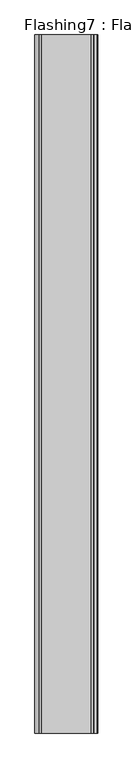
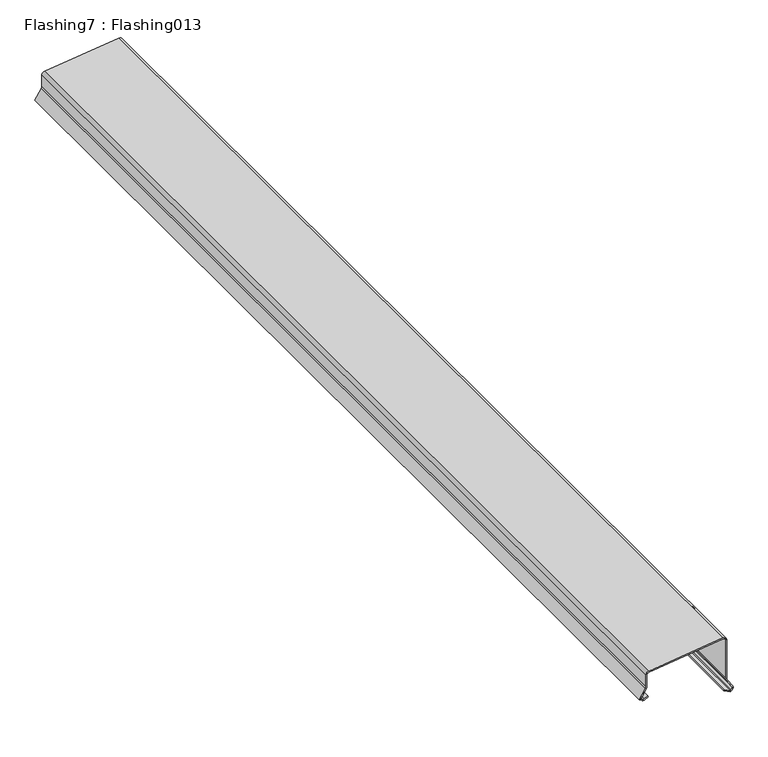
"""IFC4 building model written with IfcOpenShell, lengths in millimetres: proxy geometry, Flashing7 : Flashing013."""

from ifc_helpers import new_model, si_unit, point, frame, frame_2d, origin, place, context, project, spatial, polyline, circle_curve, trimmed, segment, composite_curve, outline, extrude, source, transform, mapped, element, save


def flashing7_flashing013_fca4859d(model_context):
    return source(origin(), model_context, "Body", "SweptSolid", [
        extrude(outline(composite_curve([segment(polyline([(40127.5360053, -9416.8782953), (40130.8867187, -9409.9548736), (40132.6869689, -9410.8261368), (40129.3362554, -9417.7495585)]), True, "CONTINUOUS"), segment(trimmed(circle_curve(frame_2d((40133.2517994, -9419.6445559)), 4.35), [point((40129.3362554, -9417.7495585))], [point((40129.5632143, -9421.9503831))], True, "CARTESIAN"), True, "CONTINUOUS"), segment(polyline([(40129.5632143, -9421.9503831), (40131.5072723, -9425.0602534), (40148.3948046, -9414.1661265)]), True, "CONTINUOUS"), segment(trimmed(circle_curve(frame_2d((40152.9212544, -9421.1828033)), 8.35), [point((40148.3948046, -9414.1661265))], [point((40152.9212544, -9412.8328033))], False, "CARTESIAN"), True, "CONTINUOUS"), segment(polyline([(40152.9212544, -9412.8328033), (40176.1640916, -9412.8328033)]), True, "CONTINUOUS"), segment(trimmed(circle_curve(frame_2d((40176.1640916, -9408.4828033)), 4.35), [point((40176.1640916, -9412.8328033))], [point((40180.4823161, -9409.0076242))], True, "CARTESIAN"), True, "CONTINUOUS"), segment(polyline([(40180.4823161, -9409.0076242), (40197.712243, -9267.2398508)]), True, "CONTINUOUS"), segment(trimmed(circle_curve(frame_2d((40193.3940184, -9266.7150298)), 4.35), [point((40197.712243, -9267.2398508))], [point((40193.3940184, -9262.3650298))], True, "CARTESIAN"), True, "CONTINUOUS"), segment(polyline([(40193.3940184, -9262.3650298), (40116.1659228, -9262.3650299)]), True, "CONTINUOUS"), segment(trimmed(circle_curve(frame_2d((40116.1659228, -9254.0150299)), 8.35), [point((40116.1659228, -9262.3650299))], [point((40111.6503228, -9261.0386939))], False, "CARTESIAN"), True, "CONTINUOUS"), segment(polyline([(40111.6503228, -9261.0386939), (40095.8098632, -9250.8546675)]), True, "CONTINUOUS"), segment(trimmed(circle_curve(frame_2d((40093.4574249, -9254.5137021)), 4.35), [point((40095.8098632, -9250.8546675))], [point((40089.7935443, -9252.1688185))], True, "CARTESIAN"), True, "CONTINUOUS"), segment(polyline([(40089.7935443, -9252.1688185), (40088.63264, -9253.9827315), (40093.9764738, -9264.6739664), (40092.1875, -9265.5681549), (40086.3359375, -9253.8611236), (40088.1090015, -9251.0907111)]), True, "CONTINUOUS"), segment(trimmed(circle_curve(frame_2d((40093.4574249, -9254.5137021)), 6.35), [point((40088.1090015, -9251.0907111))], [point((40096.8914441, -9249.1723528))], False, "CARTESIAN"), True, "CONTINUOUS"), segment(polyline([(40096.8914441, -9249.1723528), (40112.7319037, -9259.3563791)]), True, "CONTINUOUS"), segment(trimmed(circle_curve(frame_2d((40116.1659228, -9254.0150299)), 6.35), [point((40112.7319037, -9259.3563791))], [point((40116.1659228, -9260.3650299))], True, "CARTESIAN"), True, "CONTINUOUS"), segment(polyline([(40116.1659228, -9260.3650299), (40193.3940184, -9260.3650299)]), True, "CONTINUOUS"), segment(trimmed(circle_curve(frame_2d((40193.3940184, -9266.7150299)), 6.35), [point((40193.3940184, -9260.3650299))], [point((40199.6976336, -9267.4811477))], False, "CARTESIAN"), True, "CONTINUOUS"), segment(polyline([(40199.6976336, -9267.4811477), (40182.4677067, -9409.2489212)]), True, "CONTINUOUS"), segment(trimmed(circle_curve(frame_2d((40176.1640916, -9408.4828033)), 6.35), [point((40182.4677067, -9409.2489212))], [point((40176.1640916, -9414.8328033))], False, "CARTESIAN"), True, "CONTINUOUS"), segment(polyline([(40176.1640916, -9414.8328033), (40152.9212544, -9414.8328033)]), True, "CONTINUOUS"), segment(trimmed(circle_curve(frame_2d((40152.9212544, -9421.1828033)), 6.35), [point((40152.9212544, -9414.8328033))], [point((40149.4789842, -9415.8467677))], True, "CARTESIAN"), True, "CONTINUOUS"), segment(polyline([(40149.4789842, -9415.8467677), (40130.8867187, -9427.8406158), (40127.867313, -9423.0105336)]), True, "CONTINUOUS"), segment(trimmed(circle_curve(frame_2d((40133.2517994, -9419.6445559)), 6.35), [point((40127.867313, -9423.0105336))], [point((40127.5360053, -9416.8782953))], False, "CARTESIAN"), True, "CONTINUOUS")], self_intersect=False)), frame((0.0, 7982.1531721, 0.0), z_axis=(0.0, 1.0, 0.0), x_axis=(0.0, 0.0, 1.0)), (0.0, 0.0, 1.0), 2000.0),
    ])


if __name__ == "__main__":
    model = new_model("IFC4")
    model_context = context("Model", 3, world=origin())
    ifc_project = project(units=[si_unit("LENGTHUNIT", "METRE", prefix="MILLI")], contexts=[model_context])
    site = spatial("IfcSite", under=ifc_project)
    building = spatial("IfcBuilding", under=site)
    placement = place(None, origin())
    flashing7_flashing013_shape = flashing7_flashing013_fca4859d(model_context)
    element("IfcBuildingElementProxy", 1, Name="Flashing7 : Flashing013", ObjectType="Flashing7 : Flashing013", at=placement, inside=building, context=model_context, shape_type="MappedRepresentation", body=[
        mapped(flashing7_flashing013_shape, transform((0.0, 0.0, 0.0), x_axis=(1.0, 0.0, 0.0), y_axis=(0.0, 1.0, 0.0), z_axis=(0.0, 0.0, 1.0))),
    ])
    save(model, "model.ifc")

# Revit data of these elements
# Type "Flashing7 : Flashing013"
#   NameOverride = "Flashing013"
# Element 1 (IfcBuildingElementProxy, "Flashing7 : Flashing013")
#   Materials on its faces: "METAL COPING"
# Materials
#   "METAL COPING": class "Unassigned", colour RGB 128 128 128, transparency 0
